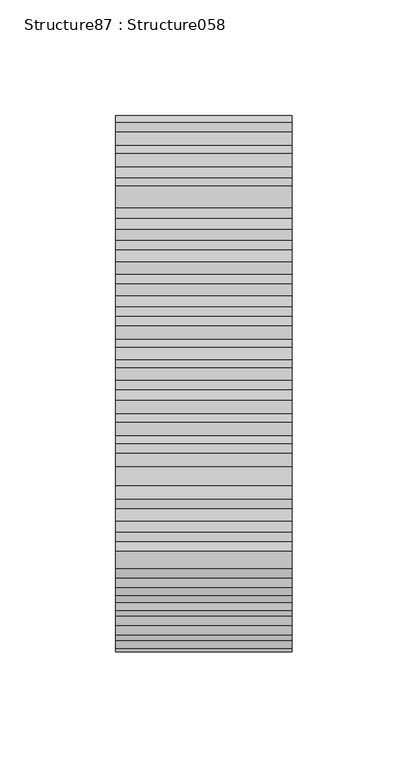
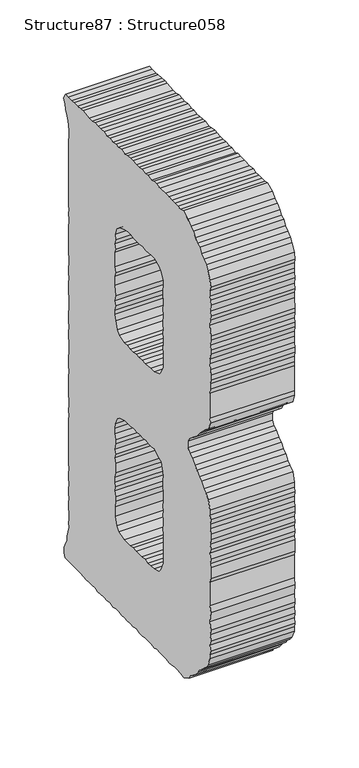
"""IFC4 building model written with IfcOpenShell, lengths in millimetres: proxy geometry, Structure87 : Structure058."""

import ifcopenshell
import ifcopenshell.guid

model = None  # the IFC model being written
_history = None  # IfcOwnerHistory: only IFC2X3 demands one
_inside = {}  # id of a spatial element -> (the spatial element, [elements in it])
_under = {}  # id of a project, library or spatial element -> (it, [spatial elements below it])
_declared = {}  # id of a project -> (the project, [libraries it declares])
_typed = {}  # id of a type object -> (the type object, [elements of that type])
_made_of = {}  # id of a material, layer set ... -> (it, [elements and type objects made of it])


def new_model(schema):
    """Start an empty IFC model of exactly this schema.

    Asked for "IFC4X3", IfcOpenShell would pick the latest addendum, in which some entities
    have other attributes; the version numbers below select the first issue.
    IFC2X3 requires an IfcOwnerHistory on every rooted entity: one is made here for all.
    """
    global model, _history
    if schema == "IFC4X3":
        model = ifcopenshell.file(schema_version=(4, 3, 0, 0))
    else:
        model = ifcopenshell.file(schema=schema)
    _inside.clear()
    _under.clear()
    _declared.clear()
    _typed.clear()
    _made_of.clear()
    _history = None
    if model.schema == "IFC2X3":
        org = make("IfcOrganization", Name="unknown")
        user = make(
            "IfcPersonAndOrganization",
            ThePerson=make("IfcPerson", FamilyName="unknown"),
            TheOrganization=org,
        )
        app = make(
            "IfcApplication",
            ApplicationDeveloper=org,
            Version="unknown",
            ApplicationFullName="unknown",
            ApplicationIdentifier="unknown",
        )
        _history = make(
            "IfcOwnerHistory",
            OwningUser=user,
            OwningApplication=app,
            ChangeAction="ADDED",
            CreationDate=0,
        )
    return model


def make(cls, **values):
    """One entity of the class cls with the attributes given. An attribute that is None is left unset."""
    return model.create_entity(
        cls, **{name: value for name, value in values.items() if value is not None}
    )


def rooted(cls, **values):
    """An entity with a GlobalId (a new one), such as an element, a storey or a relation."""
    return make(cls, GlobalId=ifcopenshell.guid.new(), OwnerHistory=_history, **values)


def si_unit(unit_type, name, prefix=None):
    """IfcSIUnit, for example si_unit("LENGTHUNIT", "METRE", prefix="MILLI")."""
    return make("IfcSIUnit", UnitType=unit_type, Prefix=prefix, Name=name)


def assignment(units):
    """IfcUnitAssignment: the units of a project."""
    return None if units is None else make("IfcUnitAssignment", Units=units)


def point(xyz):
    """IfcCartesianPoint."""
    return None if xyz is None else make("IfcCartesianPoint", Coordinates=xyz)


def direction(xyz):
    """IfcDirection."""
    return None if xyz is None else make("IfcDirection", DirectionRatios=xyz)


def frame(location, z_axis=None, x_axis=None):
    """IfcAxis2Placement3D, a coordinate frame: its origin and axes. An axis left out is left unset."""
    return make(
        "IfcAxis2Placement3D",
        Location=point(location),
        Axis=direction(z_axis),
        RefDirection=direction(x_axis),
    )


def origin():
    """The frame at (0, 0, 0) with its axes left unset."""
    return frame((0.0, 0.0, 0.0))


def place(relative_to, where):
    """IfcLocalPlacement: puts the frame where relative to a parent placement (None: the world)."""
    return make(
        "IfcLocalPlacement", PlacementRelTo=relative_to, RelativePlacement=where
    )


def context(
    kind, dimensions, precision=None, world=None, true_north=None, identifier=None
):
    """IfcGeometricRepresentationContext, for example the 3D "Model" context."""
    return make(
        "IfcGeometricRepresentationContext",
        ContextIdentifier=identifier,
        ContextType=kind,
        CoordinateSpaceDimension=dimensions,
        Precision=precision,
        WorldCoordinateSystem=world,
        TrueNorth=true_north,
    )


def project(units=None, contexts=None):
    """IfcProject with its units and contexts."""
    return rooted(
        "IfcProject",
        Name="project",
        RepresentationContexts=contexts,
        UnitsInContext=assignment(units),
    )


def spatial(cls, under=None, at=None, **own):
    """A site, building, storey or space (cls), placed at a placement, below another one or the project."""
    s = rooted(cls, ObjectPlacement=at, **own)
    if under is not None:
        _under.setdefault(under.id(), (under, []))[1].append(s)
    return s


def polyline(points):
    """IfcPolyline through the points."""
    return make("IfcPolyline", Points=[point(p) for p in points])


def outline(outer, holes=None, kind="AREA"):
    """IfcArbitraryClosedProfileDef: a profile drawn as a closed curve; with holes, ...WithVoids."""
    if holes is None:
        return make("IfcArbitraryClosedProfileDef", ProfileType=kind, OuterCurve=outer)
    return make(
        "IfcArbitraryProfileDefWithVoids",
        ProfileType=kind,
        OuterCurve=outer,
        InnerCurves=holes,
    )


def extrude(swept, where, along, depth):
    """IfcExtrudedAreaSolid: the profile swept, set in the frame where, extruded along a direction by depth."""
    return make(
        "IfcExtrudedAreaSolid",
        SweptArea=swept,
        Position=where,
        ExtrudedDirection=direction(along),
        Depth=depth,
    )


def shape(context_of_items, identifier, shape_type, items):
    """IfcShapeRepresentation: the items that make up one representation, for example the "Body"."""
    return make(
        "IfcShapeRepresentation",
        ContextOfItems=context_of_items,
        RepresentationIdentifier=identifier,
        RepresentationType=shape_type,
        Items=items,
    )


def source(mapping_origin, context_of_items, identifier, shape_type, items):
    """IfcRepresentationMap: a shape defined once, which mapped items show again and again."""
    return make(
        "IfcRepresentationMap",
        MappingOrigin=mapping_origin,
        MappedRepresentation=shape(context_of_items, identifier, shape_type, items),
    )


def transform(
    local_origin,
    x_axis=None,
    y_axis=None,
    z_axis=None,
    scale=None,
    scale2=None,
    scale3=None,
    uniform=True,
):
    """IfcCartesianTransformationOperator3D, or its non-uniform kind. x_axis, y_axis, z_axis: its Axis1, 2, 3."""
    if uniform:
        return make(
            "IfcCartesianTransformationOperator3D",
            Axis1=direction(x_axis),
            Axis2=direction(y_axis),
            LocalOrigin=point(local_origin),
            Scale=scale,
            Axis3=direction(z_axis),
        )
    return make(
        "IfcCartesianTransformationOperator3DnonUniform",
        Axis1=direction(x_axis),
        Axis2=direction(y_axis),
        LocalOrigin=point(local_origin),
        Scale=scale,
        Axis3=direction(z_axis),
        Scale2=scale2,
        Scale3=scale3,
    )


def mapped(mapping_source, mapping_target):
    """IfcMappedItem: shows the shape of a source again, moved by a transform."""
    return make(
        "IfcMappedItem", MappingSource=mapping_source, MappingTarget=mapping_target
    )


def made_of(thing, what):
    """Note that an element or type object is made of a material, layer set ...; save() writes the relation."""
    if what is not None:
        _made_of.setdefault(what.id(), (what, []))[1].append(thing)
    return thing


def element(
    cls,
    number,
    at=None,
    inside=None,
    cuts=None,
    type_object=None,
    material=None,
    context=None,
    identifier="Body",
    shape_type=None,
    held_by="IfcProductDefinitionShape",
    body=None,
    shapes=None,
    **own,
):
    """One element of the class cls, such as IfcWall. Its Tag is "e" and its number.

    at: its placement. inside: the storey or other place that contains it. cuts: it is an
    opening in that element (IfcRelVoidsElement). A single representation is given by context,
    identifier, shape_type and body (its items); several are given by shapes. held_by: the class
    of the entity that holds the representations. save() writes the other relations.
    """
    e = rooted(cls, Tag="e%d" % number, ObjectPlacement=at, **own)
    if body is not None:
        shapes = [shape(context, identifier, shape_type, body)]
    if shapes is not None:
        e.Representation = make(held_by, Representations=shapes)
    if inside is not None:
        _inside.setdefault(inside.id(), (inside, []))[1].append(e)
    if cuts is not None:
        rooted(
            "IfcRelVoidsElement", RelatingBuildingElement=cuts, RelatedOpeningElement=e
        )
    if type_object is not None:
        _typed.setdefault(type_object.id(), (type_object, []))[1].append(e)
    return made_of(e, material)


def aggregate(whole, parts):
    """IfcRelAggregates: a whole, such as a stair, and the parts it consists of."""
    return rooted("IfcRelAggregates", RelatingObject=whole, RelatedObjects=parts)


def save(model, path):
    """Write the relations noted so far, then the file.

    IfcRelAggregates (storeys below a building ...), IfcRelContainedInSpatialStructure (elements
    in a storey), IfcRelDefinesByType, IfcRelAssociatesMaterial and IfcRelDeclares: one each for
    every whole, place, type object, material and project.
    """
    for whole, parts in _under.values():
        aggregate(whole, parts)
    for where, things in _inside.values():
        rooted(
            "IfcRelContainedInSpatialStructure",
            RelatedElements=things,
            RelatingStructure=where,
        )
    for kind, things in _typed.values():
        rooted("IfcRelDefinesByType", RelatedObjects=things, RelatingType=kind)
    for what, things in _made_of.values():
        rooted("IfcRelAssociatesMaterial", RelatedObjects=things, RelatingMaterial=what)
    for by, libraries in _declared.values():
        rooted("IfcRelDeclares", RelatingContext=by, RelatedDefinitions=libraries)
    model.write(path)


def structure87_structure058_1722602e(model_context):
    return source(origin(), model_context, "Body", "SweptSolid", [
        extrude(outline(polyline([(275141.9684475, 3581.5276686), (275139.0272075, 3585.0706354), (275135.5275651, 3593.2541183), (275135.5275651, 3597.3538828), (275134.3465762, 3601.4536473), (275135.5275651, 3606.1551384), (275134.3465762, 3610.838979), (275134.9483028, 3616.69739), (275134.3465762, 3621.3732075), (275135.5275651, 3628.998288), (275134.3465762, 3638.3563415), (275135.5275651, 3644.2420307), (275135.5275651, 3666.5027089), (275134.3465762, 3670.5848228), (275134.3465762, 3681.1447249), (275134.9483028, 3684.6443673), (275134.3465762, 3689.3458585), (275135.5275651, 3694.6298211), (275134.3465762, 3698.711935), (275134.9483028, 3703.4134261), (275134.3465762, 3708.087639), (275134.3465762, 3713.3555556), (275134.9483028, 3718.0554422), (275134.9483028, 3722.7312597), (275134.3465762, 3727.4311462), (275135.5275651, 3730.9323932), (275135.5275651, 3735.6146291), (275137.868683, 3744.4158848), (275141.9684475, 3747.9428055), (275145.4905544, 3750.3015741), (275148.9885922, 3754.9854146), (275152.5331635, 3757.3185096), (275156.0312013, 3761.418274), (275159.5533082, 3764.3611187), (275163.6530727, 3768.4432325), (275167.1751795, 3770.8036057), (275170.0939551, 3774.3032481), (275170.0939551, 3780.7441306), (275167.1751795, 3785.4456218), (275162.4720838, 3788.9452642), (275158.974046, 3791.8865042), (275156.0312013, 3794.2292268), (275153.1124257, 3798.3305959), (275149.5903189, 3802.448011), (275146.0698166, 3805.3459267), (275142.5477097, 3808.290376), (275137.868683, 3811.2043377), (275134.9483028, 3819.4150989), (275135.5275651, 3823.5341187), (275135.5275651, 3847.5598618), (275134.9483028, 3851.6612309), (275134.9483028, 3856.9179152), (275134.3465762, 3861.0192843), (275134.3465762, 3865.7015202), (275134.9483028, 3870.4030114), (275135.5275651, 3875.686974), (275135.5275651, 3880.3627915), (275134.3465762, 3885.6210804), (275134.3465762, 3889.7208449), (275134.9483028, 3893.822214), (275134.3465762, 3899.1061766), (275134.3465762, 3903.2059411), (275135.5275651, 3912.5896682), (275134.9483028, 3917.8479571), (275134.3465762, 3921.9733953), (275134.9483028, 3926.6492128), (275134.3465762, 3932.4899731), (275134.9483028, 3937.1930689), (275135.5275651, 3940.718385), (275135.5275651, 3945.9766739), (275134.3465762, 3950.0940891), (275135.5275651, 3955.9348494), (275139.0272075, 3962.9774586), (275141.3891853, 3967.0788276), (275145.4905544, 3969.994394), (275149.5903189, 3972.9372387), (275151.9314368, 3977.6194746), (275155.4519391, 3979.3781211), (275158.3723193, 3982.8793681), (275161.8928215, 3987.0048063), (275165.9941906, 3989.3475288), (275170.0939551, 3993.4472933), (275177.7158265, 3996.9645864), (275181.8171956, 3995.7803883), (275185.91696, 3996.390138), (275190.6200558, 3996.390138), (275195.8799494, 3995.7803883), (275199.9797138, 3996.9645864), (275205.8413341, 3996.390138), (275214.0200032, 3996.390138), (275219.9040879, 3996.9645864), (275224.0038524, 3996.9645864), (275227.5259592, 3995.7803883), (275233.3875794, 3996.9645864), (275236.8856172, 3996.390138), (275242.7472375, 3996.9645864), (275247.4278688, 3996.390138), (275251.5276333, 3996.390138), (275256.8099913, 3996.9645864), (275260.3304935, 3996.9645864), (275265.6128515, 3996.390138), (275269.1108893, 3995.7803883), (275274.9725096, 3996.9645864), (275279.0738786, 3996.390138), (275283.1736431, 3996.390138), (275287.8767389, 3995.7803883), (275293.1366324, 3996.390138), (275297.2363969, 3995.7803883), (275302.5187549, 3996.9645864), (275307.7786485, 3996.390138), (275311.878413, 3996.390138), (275316.5815087, 3996.9645864), (275321.2605354, 3995.7803883), (275325.9636312, 3995.7803883), (275335.3232892, 3996.9645864), (275338.8453961, 3996.9645864), (275343.5244228, 3996.390138), (275349.386043, 3996.390138), (275352.9081499, 3995.7803883), (275358.7681655, 3995.7803883), (275362.8695346, 3996.390138), (275365.7883102, 3991.0788971), (275363.4487968, 3986.4046842), (275362.8695346, 3981.7208437), (275360.5300213, 3977.0209571), (275358.7681655, 3973.5197101), (275356.9854499, 3964.7361051), (275356.9854499, 3958.8776941), (275358.1664388, 3954.7506513), (275358.1664388, 3944.8165449), (275357.5871766, 3941.2912288), (275358.1664388, 3936.0345445), (275357.5871766, 3931.9058971), (275357.5871766, 3921.9733953), (275358.1664388, 3917.8479571), (275358.1664388, 3907.888177), (275357.5871766, 3902.6314927), (275358.1664388, 3899.1061766), (275357.5871766, 3893.246161), (275356.9854499, 3889.1463965), (275358.1664388, 3885.0626781), (275356.9854499, 3879.1769888), (275358.1664388, 3870.9790644), (275357.5871766, 3865.1190488), (275358.1664388, 3861.6178018), (275358.1664388, 3852.2340747), (275357.5871766, 3846.9757858), (275356.9854499, 3842.8583706), (275356.9854499, 3838.1761347), (275357.5871766, 3832.8921721), (275358.1664388, 3828.2163546), (275356.9854499, 3823.5341187), (275357.5871766, 3818.8310229), (275357.5871766, 3808.8888934), (275356.9854499, 3805.3459267), (275356.9854499, 3795.4037973), (275357.5871766, 3790.1294623), (275357.5871766, 3786.6298199), (275358.1664388, 3781.9299333), (275356.9854499, 3776.6427615), (275357.5871766, 3772.5606477), (275357.5871766, 3766.684586), (275356.9854499, 3762.0023501), (275356.9854499, 3753.2171405), (275357.5871766, 3747.9428055), (275358.1664388, 3743.2332913), (275358.1664388, 3739.1592005), (275356.9854499, 3733.8736333), (275357.5871766, 3729.7738688), (275357.5871766, 3725.0996559), (275358.1664388, 3719.8140887), (275357.5871766, 3715.1302482), (275357.5871766, 3711.6145597), (275356.9854499, 3706.3289925), (275356.9854499, 3702.229228), (275358.1664388, 3696.3884676), (275356.9854499, 3691.6869765), (275357.5871766, 3688.1873341), (275358.1664388, 3682.8857208), (275357.5871766, 3678.81163), (275358.1664388, 3674.1277895), (275358.1664388, 3668.2437048), (275357.5871766, 3664.7440624), (275358.1664388, 3658.8840468), (275357.5871766, 3655.3587307), (275357.5871766, 3650.6845178), (275358.1664388, 3645.4262289), (275356.9854499, 3640.7167147), (275358.1664388, 3636.6153456), (275358.1664388, 3631.915459), (275356.9854499, 3626.0554434), (275357.5871766, 3621.3732075), (275357.5871766, 3616.69739), (275356.9854499, 3612.5976255), (275357.5871766, 3608.4705827), (275358.1664388, 3603.2122938), (275356.9854499, 3598.5284533), (275356.9854499, 3593.2541183), (275358.1664388, 3588.5702778), (275356.9854499, 3585.0706354), (275359.9282946, 3574.5107332), (275360.5300213, 3570.4109687), (275362.2902724, 3566.3095996), (275364.6073213, 3561.025637), (275365.209048, 3555.7416744), (275363.4487968, 3551.6675836), (275339.4246583, 3551.6675836), (275335.3232892, 3551.0658569), (275330.0425358, 3550.4833855), (275325.9636312, 3551.0658569), (275320.6812732, 3551.6675836), (275316.5815087, 3551.6675836), (275312.4576752, 3550.4833855), (275307.7786485, 3550.4833855), (275303.0980172, 3551.0658569), (275297.8156592, 3550.4833855), (275292.5573702, 3551.6675836), (275287.8767389, 3550.4833855), (275283.1736431, 3551.6675836), (275279.6756053, 3551.6675836), (275274.3707829, 3551.0658569), (275269.6917562, 3551.0658569), (275266.1696493, 3550.4833855), (275260.3304935, 3551.0658569), (275256.8099913, 3550.4833855), (275251.5276333, 3551.6675836), (275246.2677397, 3550.4833855), (275242.1679752, 3550.4833855), (275236.8856172, 3551.6675836), (275228.1052214, 3551.6675836), (275222.8228634, 3550.4833855), (275219.3248256, 3551.6675836), (275214.6217299, 3551.0658569), (275205.2620718, 3551.0658569), (275199.9797138, 3550.4833855), (275195.2990825, 3551.0658569), (275191.7561158, 3551.6675836), (275187.0754845, 3551.6675836), (275182.3964578, 3551.0658569), (275176.5348376, 3550.4833855), (275168.9129662, 3554.5831499), (275166.5959173, 3558.684519), (275162.4720838, 3561.025637), (275158.974046, 3563.9412034), (275154.8502124, 3568.6426945), (275153.1124257, 3572.1423369), (275148.9885922, 3574.5107332), (275146.0698166, 3578.0103756), (275141.9684475, 3581.5276686)]), holes=[polyline([(275209.9410986, 3831.732043), (275209.3393719, 3827.6162325), (275213.4632054, 3820.015221), (275215.2009921, 3818.2309008), (275222.8228634, 3815.3313805), (275228.1052214, 3815.3313805), (275237.4648795, 3814.148787), (275241.588713, 3814.7296538), (275247.4278688, 3814.148787), (275251.5276333, 3814.7296538), (275255.6514668, 3814.148787), (275260.3304935, 3814.148787), (275265.6128515, 3814.7296538), (275269.6917562, 3814.7296538), (275277.9153542, 3817.090027), (275280.8341298, 3820.5896694), (275283.7529054, 3827.0321565), (275284.9354989, 3832.8921721), (275284.9354989, 3836.4174882), (275283.7529054, 3841.6741725), (275284.9354989, 3845.8012153), (275283.7529054, 3851.0595042), (275284.9354989, 3860.4432313), (275284.9354989, 3869.2444869), (275283.7529054, 3873.3185778), (275284.9354989, 3878.0024183), (275284.9354989, 3892.0876365), (275283.7529054, 3895.5888836), (275284.9354989, 3900.2887701), (275283.7529054, 3904.9645876), (275284.354632, 3909.6468235), (275281.413392, 3916.6653636), (275277.9153542, 3919.6066036), (275269.6917562, 3923.1319197), (275265.0111248, 3923.7079727), (275260.3304935, 3923.7079727), (275256.8099913, 3922.5494483), (275247.4278688, 3922.5494483), (275241.588713, 3923.7079727), (275237.4648795, 3922.5494483), (275232.2049859, 3923.1319197), (275227.5259592, 3923.7079727), (275223.4021257, 3923.7079727), (275215.8027188, 3920.2067257), (275213.4632054, 3917.8479571), (275209.9410986, 3910.8310217), (275209.9410986, 3905.5470591), (275210.5219654, 3900.8648231), (275210.5219654, 3896.763454), (275209.9410986, 3890.905043), (275209.9410986, 3887.9621984), (275210.5219654, 3882.7039095), (275209.3393719, 3878.0024183), (275210.5219654, 3868.6443649), (275209.3393719, 3863.9332461), (275210.5219654, 3860.4432313), (275209.3393719, 3855.1769193), (275209.3393719, 3850.4754282), (275210.5219654, 3845.1914656), (275209.3393719, 3842.2758992), (275209.3393719, 3836.4174882), (275209.9410986, 3831.732043)]), polyline([(275216.381981, 3736.7988273), (275212.8839432, 3735.0578314), (275210.5219654, 3726.8566978), (275209.3393719, 3723.3313817), (275210.5219654, 3718.6571688), (275210.5219654, 3712.7971532), (275209.3393719, 3708.087639), (275209.9410986, 3704.5879966), (275209.3393719, 3699.3136616), (275210.5219654, 3694.6298211), (275209.3393719, 3690.512406), (275210.5219654, 3685.2444894), (275209.3393719, 3681.7271964), (275209.9410986, 3676.4432338), (275210.5219654, 3672.3691429), (275209.3393719, 3667.6853024), (275209.9410986, 3662.9854159), (275209.9410986, 3658.3015753), (275209.3393719, 3653.6000842), (275209.9410986, 3648.3161216), (275209.9410986, 3639.5405396), (275213.4632054, 3631.3410106), (275215.8027188, 3628.4158166), (275222.8228634, 3626.6571701), (275228.6844837, 3626.0554434), (275233.3875794, 3625.472972), (275237.4648795, 3626.6571701), (275242.7472375, 3626.0554434), (275251.5276333, 3626.0554434), (275256.230729, 3626.6571701), (275260.9097558, 3625.472972), (275270.2934828, 3625.472972), (275278.4946164, 3628.4158166), (275281.9926542, 3631.915459), (275284.354632, 3639.5405396), (275284.354632, 3648.9258713), (275283.7529054, 3654.1841602), (275283.7529054, 3658.8840468), (275284.9354989, 3663.5598643), (275284.354632, 3667.6853024), (275284.9354989, 3671.7690209), (275284.9354989, 3676.4432338), (275283.7529054, 3681.7271964), (275283.7529054, 3690.512406), (275284.9354989, 3695.2122926), (275283.7529054, 3699.3136616), (275284.9354989, 3703.4134261), (275283.7529054, 3709.2718371), (275283.7529054, 3713.3555556), (275284.9354989, 3718.0554422), (275284.9354989, 3723.3313817), (275284.354632, 3728.0152223), (275280.8341298, 3735.0578314), (275277.9153542, 3737.400554), (275270.2934828, 3739.7416719), (275261.489018, 3739.7416719), (275255.6514668, 3740.9162424), (275251.5276333, 3739.7416719), (275246.847002, 3740.3161203), (275241.588713, 3740.3161203), (275237.4648795, 3740.9162424), (275232.2049859, 3740.3161203), (275227.5259592, 3740.3161203), (275224.0038524, 3740.9162424), (275216.381981, 3736.7988273)])]), frame((-59031.6926606, 0.0, 0.0), z_axis=(1.0, 0.0, 0.0), x_axis=(0.0, 1.0, 0.0)), (0.0, 0.0, 1.0), 76.2),
    ])


if __name__ == "__main__":
    model = new_model("IFC4")
    model_context = context("Model", 3, world=origin())
    ifc_project = project(units=[si_unit("LENGTHUNIT", "METRE", prefix="MILLI")], contexts=[model_context])
    site = spatial("IfcSite", under=ifc_project)
    building = spatial("IfcBuilding", under=site)
    placement = place(None, origin())
    structure87_structure058_shape = structure87_structure058_1722602e(model_context)
    element("IfcBuildingElementProxy", 1, Name="Structure87 : Structure058", ObjectType="Structure87 : Structure058", at=placement, inside=building, context=model_context, shape_type="MappedRepresentation", body=[
        mapped(structure87_structure058_shape, transform((0.0, 0.0, 0.0), x_axis=(1.0, 0.0, 0.0), y_axis=(0.0, 1.0, 0.0), z_axis=(0.0, 0.0, 1.0))),
    ])
    save(model, "model.ifc")

# Revit data of these elements
# Type "Structure87 : Structure058"
#   NameOverride = "Structure058"
# Element 1 (IfcBuildingElementProxy, "Structure87 : Structure058")
#   Materials on its faces: "BRUSHED ALUM. LETTERING"
# Materials
#   "BRUSHED ALUM. LETTERING": class "Unassigned", colour RGB 169 181 186, transparency 0, Cost = 0
